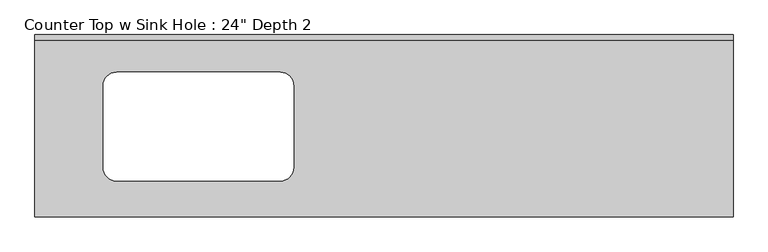
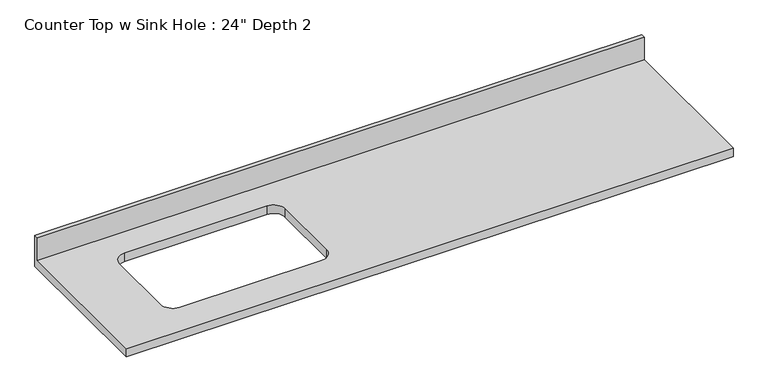
"""IFC4 building model written with IfcOpenShell, lengths in millimetres: furniture geometry."""

from ifc_helpers import new_model, si_unit, frame, origin, place, context, project, spatial, polyline, circle_curve, source, transform, mapped, element, save
from ifc_brep_helpers import plane_surface, revolved_surface, advanced_brep


def furniture_04afac51(model_context):
    return source(origin(), model_context, "Body", "AdvancedBrep", [
        advanced_brep(
        [(-1200.4622951, -679.45, 914.4), (1403.0377049, -679.45, 914.4), (1403.0377049, -19.05, 914.4), (-1200.4622951, -19.05, 914.4), (-895.6622951, -139.7, 914.4), (-286.0622951, -139.7, 914.4), (-235.2622951, -190.5, 914.4), (-235.2622951, -495.3, 914.4), (-286.0622951, -546.1, 914.4), (-895.6622951, -546.1, 914.4), (-946.4622951, -495.3, 914.4), (-946.4622951, -190.5, 914.4), (1403.0377049, 0.0, 876.3), (1403.0377049, -679.45, 876.3), (-1200.4622951, -679.45, 876.3), (-1200.4622951, 0.0, 876.3), (-286.0622951, -139.7, 876.3), (-895.6622951, -139.7, 876.3), (-946.4622951, -190.5, 876.3), (-946.4622951, -495.3, 876.3), (-895.6622951, -546.1, 876.3), (-286.0622951, -546.1, 876.3), (-235.2622951, -495.3, 876.3), (-235.2622951, -190.5, 876.3), (-1200.4622951, 0.0, 1016.0), (1403.0377049, 0.0, 1016.0), (-1200.4622951, -19.05, 1016.0), (1403.0377049, -19.05, 1016.0)],
        [
            (0, 1),
            (1, 2),
            (2, 3),
            (3, 0),
            (4, 5),
            (5, 6, circle_curve(frame((-286.0622951, -190.5, 914.4), z_axis=(0.0, 0.0, -1.0), x_axis=(1.0, 0.0, 0.0)), 50.8)),
            (6, 7),
            (7, 8, circle_curve(frame((-286.0622951, -495.3, 914.4), z_axis=(0.0, 0.0, -1.0), x_axis=(1.0, 0.0, 0.0)), 50.8)),
            (8, 9),
            (9, 10, circle_curve(frame((-895.6622951, -495.3, 914.4), z_axis=(0.0, 0.0, -1.0), x_axis=(1.0, 0.0, 0.0)), 50.8)),
            (10, 11),
            (11, 4, circle_curve(frame((-895.6622951, -190.5, 914.4), z_axis=(0.0, 0.0, -1.0), x_axis=(1.0, 0.0, 0.0)), 50.8)),
            (12, 13),
            (13, 14),
            (14, 15),
            (15, 12),
            (16, 17),
            (17, 18, circle_curve(frame((-895.6622951, -190.5, 876.3), z_axis=(0.0, 0.0, 1.0), x_axis=(1.0, 0.0, 0.0)), 50.8)),
            (18, 19),
            (19, 20, circle_curve(frame((-895.6622951, -495.3, 876.3), z_axis=(0.0, 0.0, 1.0), x_axis=(1.0, 0.0, 0.0)), 50.8)),
            (20, 21),
            (21, 22, circle_curve(frame((-286.0622951, -495.3, 876.3), z_axis=(0.0, 0.0, 1.0), x_axis=(1.0, 0.0, 0.0)), 50.8)),
            (22, 23),
            (23, 16, circle_curve(frame((-286.0622951, -190.5, 876.3), z_axis=(0.0, 0.0, 1.0), x_axis=(1.0, 0.0, 0.0)), 50.8)),
            (15, 24),
            (24, 25),
            (25, 12),
            (14, 0),
            (3, 26),
            (26, 24),
            (13, 1),
            (25, 27),
            (27, 2),
            (26, 27),
            (4, 17),
            (16, 5),
            (11, 18),
            (10, 19),
            (9, 20),
            (8, 21),
            (7, 22),
            (6, 23),
        ],
        [
            plane_surface(frame((-1200.4622951, 0.0, 914.4), z_axis=(0.0, 0.0, 1.0), x_axis=(-1.0, 0.0, 0.0))),
            plane_surface(frame((-1200.4622951, 0.0, 876.3), z_axis=(0.0, 0.0, -1.0), x_axis=(1.0, 0.0, 0.0))),
            plane_surface(frame((1403.0377049, 0.0, 914.4), z_axis=(0.0, 1.0, 0.0), x_axis=(0.0, 0.0, -1.0))),
            plane_surface(frame((-1200.4622951, 0.0, 914.4), z_axis=(-1.0, 0.0, 0.0), x_axis=(0.0, 0.0, -1.0))),
            plane_surface(frame((-1200.4622951, -679.45, 914.4), z_axis=(0.0, -1.0, 0.0), x_axis=(0.0, 0.0, -1.0))),
            plane_surface(frame((1403.0377049, -679.45, 914.4), z_axis=(1.0, 0.0, 0.0), x_axis=(0.0, 0.0, -1.0))),
            plane_surface(frame((-1200.4622951, 0.0, 1016.0), z_axis=(0.0, 0.0, 1.0), x_axis=(0.0, -1.0, 0.0))),
            plane_surface(frame((-1200.4622951, -19.05, 1016.0), z_axis=(0.0, -1.0, 0.0), x_axis=(0.0, 0.0, -1.0))),
            plane_surface(frame((-286.0622951, -139.7, 914.4), z_axis=(0.0, -1.0, 0.0), x_axis=(0.0, 0.0, -1.0))),
            revolved_surface(polyline([(-844.8622951000001, -190.5, 914.4), (-844.8622951000001, -190.5, 876.3)]), (-895.6622951, -190.5, 876.3), (0.0, 0.0, 1.0)),
            plane_surface(frame((-946.4622951, -190.5, 914.4), z_axis=(1.0, 0.0, 0.0), x_axis=(0.0, 0.0, -1.0))),
            revolved_surface(polyline([(-844.8622951000001, -495.3, 914.4), (-844.8622951000001, -495.3, 876.3)]), (-895.6622951, -495.3, 876.3), (0.0, 0.0, 1.0)),
            plane_surface(frame((-895.6622951, -546.1, 914.4), z_axis=(0.0, 1.0, 0.0), x_axis=(0.0, 0.0, -1.0))),
            revolved_surface(polyline([(-235.26229509999996, -495.3, 914.4), (-235.26229509999996, -495.3, 876.3)]), (-286.0622951, -495.3, 876.3), (0.0, 0.0, 1.0)),
            plane_surface(frame((-235.2622951, -495.3, 914.4), z_axis=(-1.0, 0.0, 0.0), x_axis=(0.0, 0.0, -1.0))),
            revolved_surface(polyline([(-235.26229509999996, -190.5, 914.4), (-235.26229509999996, -190.5, 876.3)]), (-286.0622951, -190.5, 876.3), (0.0, 0.0, 1.0)),
        ],
        [
            (0, [[1, 2, 3, 4], [5, 6, 7, 8, 9, 10, 11, 12]]),
            (1, [[13, 14, 15, 16], [17, 18, 19, 20, 21, 22, 23, 24]]),
            (2, [[-16, 25, 26, 27]]),
            (3, [[-15, 28, -4, 29, 30, -25]]),
            (4, [[-1, -28, -14, 31]]),
            (5, [[-13, -27, 32, 33, -2, -31]]),
            (6, [[-30, 34, -32, -26]]),
            (7, [[-34, -29, -3, -33]]),
            (8, [[35, -17, 36, -5]]),
            (9, [[-35, -12, 37, -18]]),
            (10, [[-37, -11, 38, -19]]),
            (11, [[-38, -10, 39, -20]]),
            (12, [[-39, -9, 40, -21]]),
            (13, [[-40, -8, 41, -22]]),
            (14, [[-41, -7, 42, -23]]),
            (15, [[-36, -24, -42, -6]]),
        ],
    ),
    ])


if __name__ == "__main__":
    model = new_model("IFC4")
    model_context = context("Model", 3, world=origin())
    ifc_project = project(units=[si_unit("LENGTHUNIT", "METRE", prefix="MILLI")], contexts=[model_context])
    site = spatial("IfcSite", under=ifc_project)
    building = spatial("IfcBuilding", under=site)
    placement = place(None, origin())
    furniture_shape = furniture_04afac51(model_context)
    element("IfcFurniture", 1, ObjectType="Counter Top w Sink Hole : 24\" Depth 2", at=placement, inside=building, context=model_context, shape_type="MappedRepresentation", body=[
        mapped(furniture_shape, transform((0.0, 0.0, 0.0), x_axis=(1.0, 0.0, 0.0), y_axis=(0.0, 1.0, 0.0), z_axis=(0.0, 0.0, 1.0))),
    ])
    save(model, "model.ifc")

# Revit data of these elements
# Type "Counter Top w Sink Hole : 24\" Depth 2"
#   Assembly Code = "C1030400"
#   Counter Thickness = 0' - 1 1/2"
#   Depth = 2' - 2 3/4"
#   Height = 3' - 0"
#   Length [instance default] = 8' - 0"
#   Sink Location [instance default] = 2' - 0"
#   Sink Location To Wall [instance default] = 0' - 6"
#   Sink Opening Depth [instance default] = 1' - 3"
#   Sink Opening Width [instance default] = 2' - 3"
#   Counter Top Material = none
# Element 1 (IfcFurniture, "Counter Top w Sink Hole : 24\" Depth 2")
#   Length = 8' - 6 1/2"
#   Materials on its faces: "Counter Top"
# Materials
#   "Counter Top": class "Wood", colour RGB 226 177 128, transparency 0
